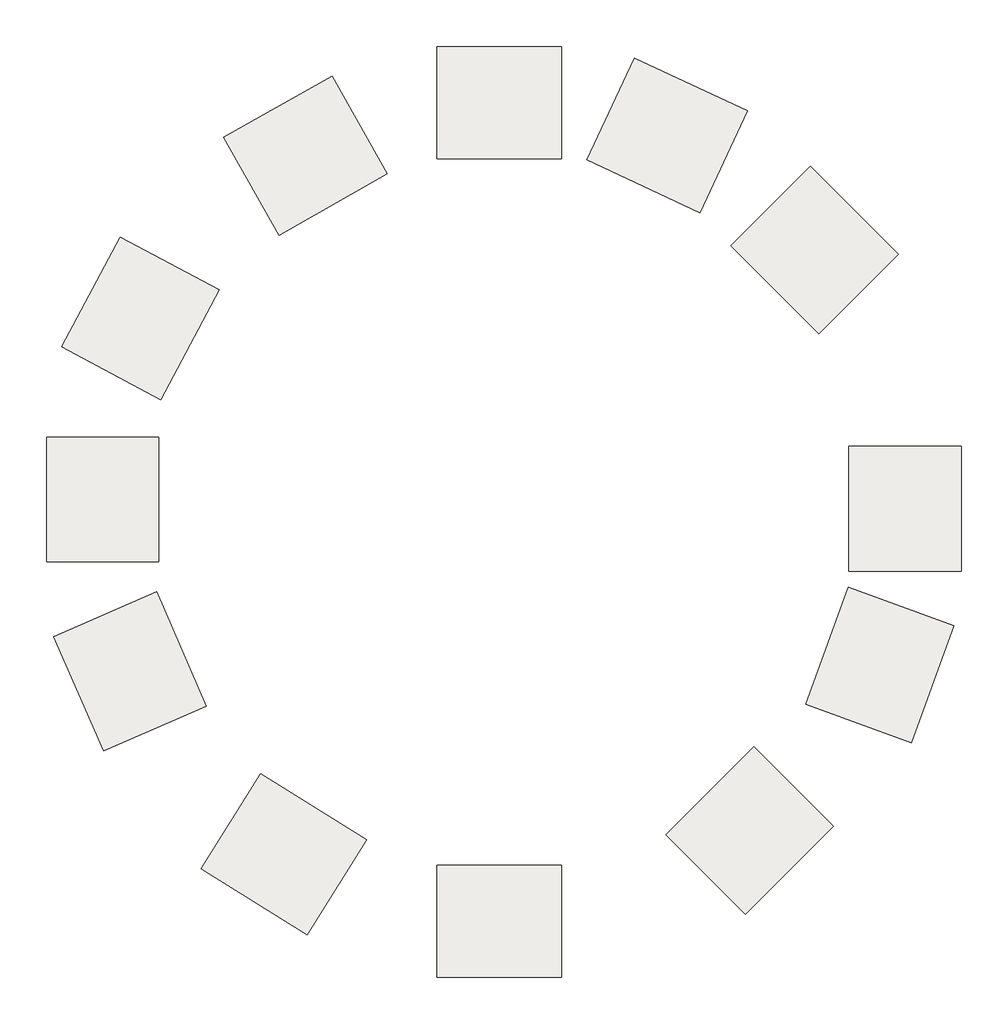
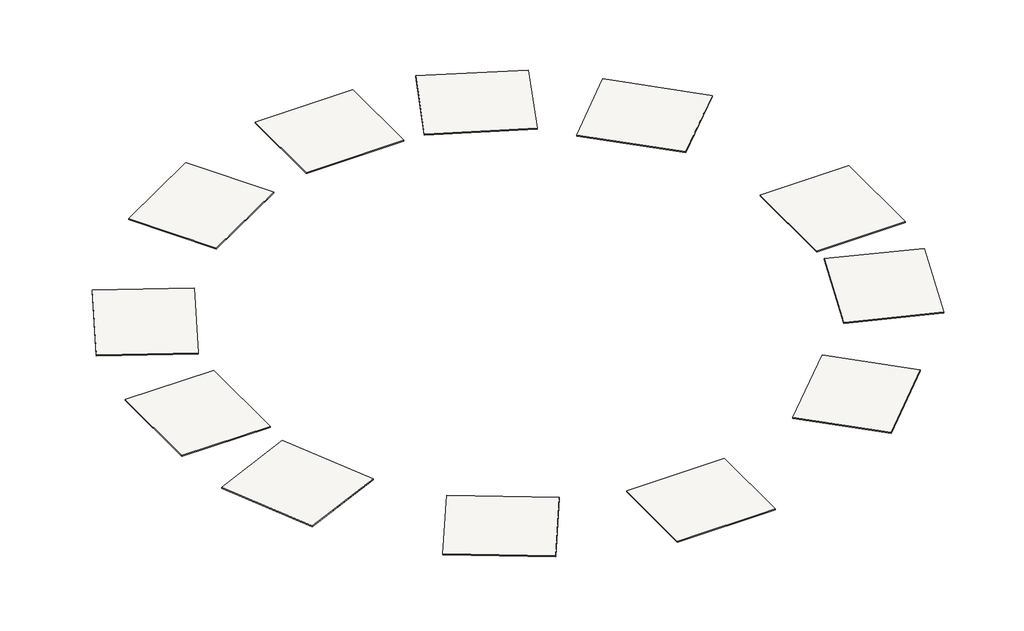
# One storey: 12 slabs.
"""IFC4 building model written with IfcOpenShell, lengths in millimetres."""

from ifc_helpers import new_model, si_unit, frame, origin, place, context, project, spatial, polyline, outline, extrude, element, save

model = new_model("IFC4")

# Units and contexts
model_context = context("Model", 3, world=origin())
ifc_project = project(units=[si_unit("LENGTHUNIT", "METRE", prefix="MILLI")], contexts=[model_context])

# Site, building, storey
site = spatial("IfcSite", under=ifc_project)
building = spatial("IfcBuilding", under=site)
storey = spatial("IfcBuildingStorey", under=building, Name="03 этаж_+6.600", Elevation=6600.0)

# Slabs
placement = place(None, origin())
element("IfcSlab", 1, ObjectType="Перекрытие_Б220", at=placement, inside=storey, context=model_context, shape_type="SweptSolid", body=[
    extrude(outline(polyline([(20190.0, 18190.0), (20190.0, -190.0), (-190.0, -190.0), (-190.0, 18190.0), (20190.0, 18190.0)])), frame((0.0, 0.0, 6380.0), z_axis=(0.0, 0.0, 1.0), x_axis=(1.0, 0.0, 0.0)), (0.0, 0.0, 1.0), 220.0),
])
element("IfcSlab", 2, ObjectType="Перекрытие_Б220", at=placement, inside=storey, context=model_context, shape_type="SweptSolid", body=[
    extrude(outline(polyline([(85658.0374315, -67658.0374315), (67278.0374315, -67658.0374315), (67278.0374315, -47278.0374315), (85658.0374315, -47278.0374315), (85658.0374315, -67658.0374315)])), frame((0.0, 0.0, 6380.0), z_axis=(0.0, 0.0, 1.0), x_axis=(1.0, 0.0, 0.0)), (0.0, 0.0, 1.0), 220.0),
])
element("IfcSlab", 3, ObjectType="Перекрытие_Б220", at=placement, inside=storey, context=model_context, shape_type="SweptSolid", body=[
    extrude(outline(polyline([(-190.0, -134190.0), (-190.0, -115810.0), (20190.0, -115810.0), (20190.0, -134190.0), (-190.0, -134190.0)])), frame((0.0, 0.0, 6380.0), z_axis=(0.0, 0.0, 1.0), x_axis=(1.0, 0.0, 0.0)), (0.0, 0.0, 1.0), 220.0),
])
element("IfcSlab", 4, ObjectType="Перекрытие_Б220", at=placement, inside=storey, context=model_context, shape_type="SweptSolid", body=[
    extrude(outline(polyline([(-64145.4225187, -45750.266627), (-45765.4225187, -45750.266627), (-45765.4225187, -66130.266627), (-64145.4225187, -66130.266627), (-64145.4225187, -45750.266627)])), frame((0.0, 0.0, 6380.0), z_axis=(0.0, 0.0, 1.0), x_axis=(1.0, 0.0, 0.0)), (0.0, 0.0, 1.0), 220.0),
])
element("IfcSlab", 5, ObjectType="Перекрытие_Б220", at=placement, inside=storey, context=model_context, shape_type="SweptSolid", body=[
    extrude(outline(polyline([(50604.6993118, 7679.8366052), (42836.975661, -8978.1005205), (24366.4229612, -365.1403463), (32134.146612, 16292.7967795), (50604.6993118, 7679.8366052)])), frame((0.0, 0.0, 6380.0), z_axis=(0.0, 0.0, 1.0), x_axis=(1.0, 0.0, 0.0)), (0.0, 0.0, 1.0), 220.0),
])
element("IfcSlab", 6, ObjectType="Перекрытие_Б220", at=placement, inside=storey, context=model_context, shape_type="SweptSolid", body=[
    extrude(outline(polyline([(75363.2732805, -15796.3477004), (62366.6506423, -28792.9703386), (47955.8144417, -14382.134138), (60952.4370799, -1385.5114998), (75363.2732805, -15796.3477004)])), frame((0.0, 0.0, 6380.0), z_axis=(0.0, 0.0, 1.0), x_axis=(1.0, 0.0, 0.0)), (0.0, 0.0, 1.0), 220.0),
])
element("IfcSlab", 7, ObjectType="Перекрытие_Б220", at=placement, inside=storey, context=model_context, shape_type="SweptSolid", body=[
    extrude(outline(polyline([(77505.7140028, -95774.5505936), (60234.1636327, -89488.2203593), (67204.5341537, -70337.2847476), (84476.0845237, -76623.614982), (77505.7140028, -95774.5505936)])), frame((0.0, 0.0, 6380.0), z_axis=(0.0, 0.0, 1.0), x_axis=(1.0, 0.0, 0.0)), (0.0, 0.0, 1.0), 220.0),
])
element("IfcSlab", 8, ObjectType="Перекрытие_Б220", at=placement, inside=storey, context=model_context, shape_type="SweptSolid", body=[
    extrude(outline(polyline([(50314.4806804, -123839.0699449), (37317.8580422, -110842.4473067), (51728.6942428, -96431.6111061), (64725.316881, -109428.2337443), (50314.4806804, -123839.0699449)])), frame((0.0, 0.0, 6380.0), z_axis=(0.0, 0.0, 1.0), x_axis=(1.0, 0.0, 0.0)), (0.0, 0.0, 1.0), 220.0),
])
element("IfcSlab", 9, ObjectType="Перекрытие_Б220", at=placement, inside=storey, context=model_context, shape_type="SweptSolid", body=[
    extrude(outline(polyline([(-38793.1496827, -116435.1817812), (-29053.2336061, -100848.0577739), (-11770.0134064, -111647.812379), (-21509.929483, -127234.9363863), (-38793.1496827, -116435.1817812)])), frame((0.0, 0.0, 6380.0), z_axis=(0.0, 0.0, 1.0), x_axis=(1.0, 0.0, 0.0)), (0.0, 0.0, 1.0), 220.0),
])
element("IfcSlab", 10, ObjectType="Перекрытие_Б220", at=placement, inside=storey, context=model_context, shape_type="SweptSolid", body=[
    extrude(outline(polyline([(-62945.9679826, -78412.0948274), (-46090.4038154, -71083.0869405), (-37963.8977907, -89772.7712565), (-54819.4619579, -97101.7791433), (-62945.9679826, -78412.0948274)])), frame((0.0, 0.0, 6380.0), z_axis=(0.0, 0.0, 1.0), x_axis=(1.0, 0.0, 0.0)), (0.0, 0.0, 1.0), 220.0),
])
element("IfcSlab", 11, ObjectType="Перекрытие_Б220", at=placement, inside=storey, context=model_context, shape_type="SweptSolid", body=[
    extrude(outline(polyline([(-52076.3458903, -12986.4619107), (-35847.7691336, -21615.3492347), (-45415.5995832, -39609.8211772), (-61644.1763399, -30980.9338532), (-52076.3458903, -12986.4619107)])), frame((0.0, 0.0, 6380.0), z_axis=(0.0, 0.0, 1.0), x_axis=(1.0, 0.0, 0.0)), (0.0, 0.0, 1.0), 220.0),
])
element("IfcSlab", 12, ObjectType="Перекрытие_Б220", at=placement, inside=storey, context=model_context, shape_type="SweptSolid", body=[
    extrude(outline(polyline([(-17402.3317509, 13342.9287563), (-8351.5867162, -2654.2089351), (-26089.4357995, -12689.80109), (-35140.1808342, 3307.3366013), (-17402.3317509, 13342.9287563)])), frame((0.0, 0.0, 6380.0), z_axis=(0.0, 0.0, 1.0), x_axis=(1.0, 0.0, 0.0)), (0.0, 0.0, 1.0), 220.0),
])

save(model, "model.ifc")

# Revit data of these elements
# Type "Перекрытие_Б220"
#   Model = "АР"
#   Function = 0
#   Layers, outside or top first: 220 mm "Бетон B20" (function 1)
# Element 1 (IfcSlab, "Перекрытие_Б220")
#   Height Offset From Level = 0 mm
#   Phase Created = 1
#   Materials on its faces: "Бетон B20"
# Element 2 (IfcSlab, "Перекрытие_Б220")
#   built-in parameter 1001955 = -1.5708 (stored number, unit not read)
#   Height Offset From Level = 0 mm
#   Phase Created = 1
#   Materials on its faces: "Бетон B20"
# Element 3 (IfcSlab, "Перекрытие_Б220")
#   built-in parameter 1001955 = 3.14159 (stored number, unit not read)
#   Height Offset From Level = 0 mm
#   Phase Created = 1
#   Materials on its faces: "Бетон B20"
# Element 4 (IfcSlab, "Перекрытие_Б220")
#   built-in parameter 1001955 = 1.5708 (stored number, unit not read)
#   Height Offset From Level = 0 mm
#   Phase Created = 1
#   Materials on its faces: "Бетон B20"
# Element 5 (IfcSlab, "Перекрытие_Б220")
#   built-in parameter 1001955 = -0.436332 (stored number, unit not read)
#   Height Offset From Level = 0 mm
#   Phase Created = 1
#   Materials on its faces: "Бетон B20"
# Element 6 (IfcSlab, "Перекрытие_Б220")
#   built-in parameter 1001955 = -0.785398 (stored number, unit not read)
#   Height Offset From Level = 0 mm
#   Phase Created = 1
#   Materials on its faces: "Бетон B20"
# Element 7 (IfcSlab, "Перекрытие_Б220")
#   built-in parameter 1001955 = -1.91986 (stored number, unit not read)
#   Height Offset From Level = 0 mm
#   Phase Created = 1
#   Materials on its faces: "Бетон B20"
# Element 8 (IfcSlab, "Перекрытие_Б220")
#   built-in parameter 1001955 = -2.35619 (stored number, unit not read)
#   Height Offset From Level = 0 mm
#   Phase Created = 1
#   Materials on its faces: "Бетон B20"
# Element 9 (IfcSlab, "Перекрытие_Б220")
#   built-in parameter 1001955 = 2.58309 (stored number, unit not read)
#   Height Offset From Level = 0 mm
#   Phase Created = 1
#   Materials on its faces: "Бетон B20"
# Element 10 (IfcSlab, "Перекрытие_Б220")
#   built-in parameter 1001955 = 1.98095 (stored number, unit not read)
#   Height Offset From Level = 0 mm
#   Phase Created = 1
#   Materials on its faces: "Бетон B20"
# Element 11 (IfcSlab, "Перекрытие_Б220")
#   built-in parameter 1001955 = 1.0821 (stored number, unit not read)
#   Height Offset From Level = 0 mm
#   Phase Created = 1
#   Materials on its faces: "Бетон B20"
# Element 12 (IfcSlab, "Перекрытие_Б220")
#   built-in parameter 1001955 = 0.514872 (stored number, unit not read)
#   Height Offset From Level = 0 mm
#   Phase Created = 1
#   Materials on its faces: "Бетон B20"
# Materials
#   "Бетон B20": class "Бетон", colour RGB 120 120 120, transparency 0, Manufacturer = "Альтек", Description = "Бетон, 20 МПа", Cost = 0
